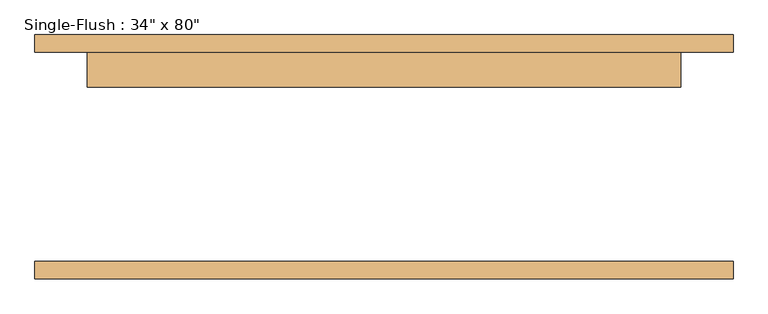
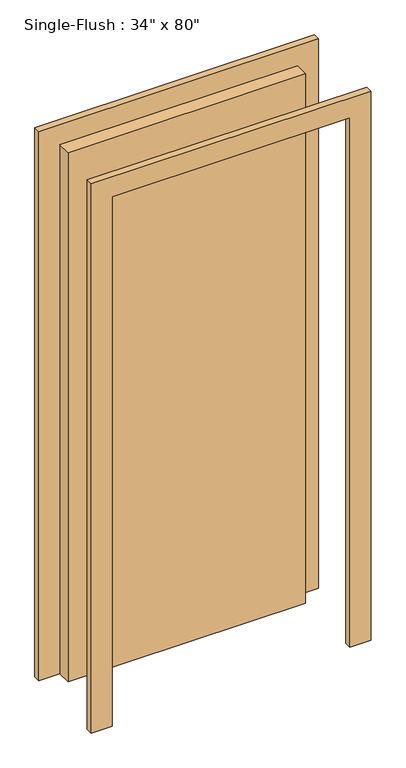
"""IFC4 building model written with IfcOpenShell, lengths in millimetres: door geometry."""

from ifc_helpers import new_model, si_unit, frame, origin, origin_with_axes, place, context, project, spatial, polyline, outline, extrude, source, transform, mapped, element, save


def door_93553381(model_context):
    return source(origin(), model_context, "Body", "SweptSolid", [
        extrude(outline(polyline([(2108.2, -508.0), (0.0, -508.0), (0.0, -431.8), (2032.0, -431.8), (2032.0, 431.8), (0.0, 431.8), (0.0, 508.0), (2108.2, 508.0), (2108.2, -508.0)])), frame((0.0, 152.4, 0.0), z_axis=(0.0, 1.0, 0.0), x_axis=(0.0, 0.0, 1.0)), (0.0, 0.0, 1.0), 25.4),
        extrude(outline(polyline([(2108.2, 508.0), (2108.2, -508.0), (0.0, -508.0), (0.0, -431.8), (2032.0, -431.8), (2032.0, 431.8), (0.0, 431.8), (0.0, 508.0), (2108.2, 508.0)])), frame((0.0, -177.8, 0.0), z_axis=(0.0, 1.0, 0.0), x_axis=(0.0, 0.0, 1.0)), (0.0, 0.0, 1.0), 25.4),
        extrude(outline(polyline([(431.8, 101.6), (-431.8, 101.6), (-431.8, 152.4), (431.8, 152.4), (431.8, 101.6)])), origin_with_axes(), (0.0, 0.0, 1.0), 2032.0),
    ])


if __name__ == "__main__":
    model = new_model("IFC4")
    model_context = context("Model", 3, world=origin())
    ifc_project = project(units=[si_unit("LENGTHUNIT", "METRE", prefix="MILLI")], contexts=[model_context])
    site = spatial("IfcSite", under=ifc_project)
    building = spatial("IfcBuilding", under=site)
    placement = place(None, origin())
    door_shape = door_93553381(model_context)
    element("IfcDoor", 1, ObjectType="Single-Flush : 34\" x 80\"", at=placement, inside=building, context=model_context, shape_type="MappedRepresentation", body=[
        mapped(door_shape, transform((0.0, 0.0, 0.0), x_axis=(1.0, 0.0, 0.0), y_axis=(0.0, 1.0, 0.0), z_axis=(0.0, 0.0, 1.0))),
    ])
    save(model, "model.ifc")

# Revit data of these elements
# Type "Single-Flush : 34\" x 80\""
#   Type Mark = "7"
#   Construction Type Id = "MDOOR"
#   Assembly Code = "C1020"
#   Analytic Construction = "Metal"
#   Thickness = 0' - 2"
#   Heat Transfer Coefficient (U) = 0.651978 BTU/(h·ft²·°F)
#   Height = 6' - 8"
#   Trim Projection Ext = 0' - 1"
#   Trim Projection Int = 0' - 1"
#   Trim Width = 0' - 3"
#   Width = 2' - 10"
#   Define Thermal Properties by = 1
#   Define Thermal Properties by = 1
#   Door Material = Door - Panel
#   Frame Material = Door - Frame
#   Visual Light Transmittance = 0
#   Solar Heat Gain Coefficient = 0
#   Function = (empty or 0)
#   Wall Closure = (empty or 0)
# Element 1 (IfcDoor, "Single-Flush : 34\" x 80\"")
#   Materials on its faces: "Door - Frame", "Door - Panel"
# Materials
#   "Door - Panel": class "Wood", colour RGB 210 159 95, transparency 0, Cost = 0
#   "Door - Frame": class "Miscellaneous", colour RGB 118 70 51, transparency 0, Cost = 0
